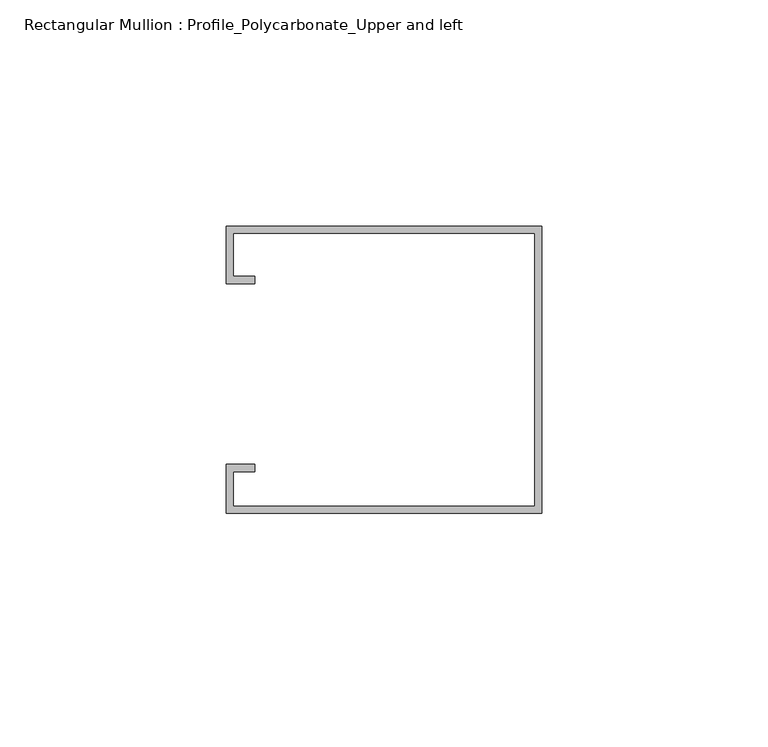
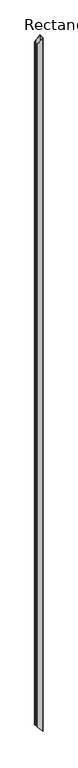
"""IFC4 building model written with IfcOpenShell, lengths in millimetres: member geometry, Rectangular Mullion : Profile_Polycarbonate_Upper and left."""

import ifcopenshell
import ifcopenshell.guid

model = None  # the IFC model being written
_history = None  # IfcOwnerHistory: only IFC2X3 demands one
_inside = {}  # id of a spatial element -> (the spatial element, [elements in it])
_under = {}  # id of a project, library or spatial element -> (it, [spatial elements below it])
_declared = {}  # id of a project -> (the project, [libraries it declares])
_typed = {}  # id of a type object -> (the type object, [elements of that type])
_made_of = {}  # id of a material, layer set ... -> (it, [elements and type objects made of it])


def new_model(schema):
    """Start an empty IFC model of exactly this schema.

    Asked for "IFC4X3", IfcOpenShell would pick the latest addendum, in which some entities
    have other attributes; the version numbers below select the first issue.
    IFC2X3 requires an IfcOwnerHistory on every rooted entity: one is made here for all.
    """
    global model, _history
    if schema == "IFC4X3":
        model = ifcopenshell.file(schema_version=(4, 3, 0, 0))
    else:
        model = ifcopenshell.file(schema=schema)
    _inside.clear()
    _under.clear()
    _declared.clear()
    _typed.clear()
    _made_of.clear()
    _history = None
    if model.schema == "IFC2X3":
        org = make("IfcOrganization", Name="unknown")
        user = make(
            "IfcPersonAndOrganization",
            ThePerson=make("IfcPerson", FamilyName="unknown"),
            TheOrganization=org,
        )
        app = make(
            "IfcApplication",
            ApplicationDeveloper=org,
            Version="unknown",
            ApplicationFullName="unknown",
            ApplicationIdentifier="unknown",
        )
        _history = make(
            "IfcOwnerHistory",
            OwningUser=user,
            OwningApplication=app,
            ChangeAction="ADDED",
            CreationDate=0,
        )
    return model


def make(cls, **values):
    """One entity of the class cls with the attributes given. An attribute that is None is left unset."""
    return model.create_entity(
        cls, **{name: value for name, value in values.items() if value is not None}
    )


def rooted(cls, **values):
    """An entity with a GlobalId (a new one), such as an element, a storey or a relation."""
    return make(cls, GlobalId=ifcopenshell.guid.new(), OwnerHistory=_history, **values)


def si_unit(unit_type, name, prefix=None):
    """IfcSIUnit, for example si_unit("LENGTHUNIT", "METRE", prefix="MILLI")."""
    return make("IfcSIUnit", UnitType=unit_type, Prefix=prefix, Name=name)


def assignment(units):
    """IfcUnitAssignment: the units of a project."""
    return None if units is None else make("IfcUnitAssignment", Units=units)


def point(xyz):
    """IfcCartesianPoint."""
    return None if xyz is None else make("IfcCartesianPoint", Coordinates=xyz)


def direction(xyz):
    """IfcDirection."""
    return None if xyz is None else make("IfcDirection", DirectionRatios=xyz)


def frame(location, z_axis=None, x_axis=None):
    """IfcAxis2Placement3D, a coordinate frame: its origin and axes. An axis left out is left unset."""
    return make(
        "IfcAxis2Placement3D",
        Location=point(location),
        Axis=direction(z_axis),
        RefDirection=direction(x_axis),
    )


def origin():
    """The frame at (0, 0, 0) with its axes left unset."""
    return frame((0.0, 0.0, 0.0))


def place(relative_to, where):
    """IfcLocalPlacement: puts the frame where relative to a parent placement (None: the world)."""
    return make(
        "IfcLocalPlacement", PlacementRelTo=relative_to, RelativePlacement=where
    )


def context(
    kind, dimensions, precision=None, world=None, true_north=None, identifier=None
):
    """IfcGeometricRepresentationContext, for example the 3D "Model" context."""
    return make(
        "IfcGeometricRepresentationContext",
        ContextIdentifier=identifier,
        ContextType=kind,
        CoordinateSpaceDimension=dimensions,
        Precision=precision,
        WorldCoordinateSystem=world,
        TrueNorth=true_north,
    )


def project(units=None, contexts=None):
    """IfcProject with its units and contexts."""
    return rooted(
        "IfcProject",
        Name="project",
        RepresentationContexts=contexts,
        UnitsInContext=assignment(units),
    )


def spatial(cls, under=None, at=None, **own):
    """A site, building, storey or space (cls), placed at a placement, below another one or the project."""
    s = rooted(cls, ObjectPlacement=at, **own)
    if under is not None:
        _under.setdefault(under.id(), (under, []))[1].append(s)
    return s


def faces_of(points, faces, orient=None, outer=None):
    """IfcFace entities. A face is a list of loops; a loop is a list of indices into points, from 0.

    orient and outer hold one flag for each loop. By default every Orientation is true, the
    first loop of a face is its IfcFaceOuterBound and the others are IfcFaceBound.
    """
    made = []
    for i, loops in enumerate(faces):
        bounds = []
        for j, loop in enumerate(loops):
            is_outer = j == 0 if outer is None else outer[i][j]
            bounds.append(
                make(
                    "IfcFaceOuterBound" if is_outer else "IfcFaceBound",
                    Bound=make("IfcPolyLoop", Polygon=[points[k] for k in loop]),
                    Orientation=True if orient is None else orient[i][j],
                )
            )
        made.append(make("IfcFace", Bounds=bounds))
    return made


def faceted_brep(points, faces, orient=None, outer=None, voids=None):
    """IfcFacetedBrep: a solid bounded by flat faces; with voids (closed shells), ...WithVoids."""
    shared = [point(p) for p in points]
    hull = make("IfcClosedShell", CfsFaces=faces_of(shared, faces, orient, outer))
    if voids is None:
        return make("IfcFacetedBrep", Outer=hull)
    return make(
        "IfcFacetedBrepWithVoids",
        Outer=hull,
        Voids=[
            make(cls, CfsFaces=faces_of(shared, fs, o, b)) for cls, fs, o, b in voids
        ],
    )


def shape(context_of_items, identifier, shape_type, items):
    """IfcShapeRepresentation: the items that make up one representation, for example the "Body"."""
    return make(
        "IfcShapeRepresentation",
        ContextOfItems=context_of_items,
        RepresentationIdentifier=identifier,
        RepresentationType=shape_type,
        Items=items,
    )


def source(mapping_origin, context_of_items, identifier, shape_type, items):
    """IfcRepresentationMap: a shape defined once, which mapped items show again and again."""
    return make(
        "IfcRepresentationMap",
        MappingOrigin=mapping_origin,
        MappedRepresentation=shape(context_of_items, identifier, shape_type, items),
    )


def transform(
    local_origin,
    x_axis=None,
    y_axis=None,
    z_axis=None,
    scale=None,
    scale2=None,
    scale3=None,
    uniform=True,
):
    """IfcCartesianTransformationOperator3D, or its non-uniform kind. x_axis, y_axis, z_axis: its Axis1, 2, 3."""
    if uniform:
        return make(
            "IfcCartesianTransformationOperator3D",
            Axis1=direction(x_axis),
            Axis2=direction(y_axis),
            LocalOrigin=point(local_origin),
            Scale=scale,
            Axis3=direction(z_axis),
        )
    return make(
        "IfcCartesianTransformationOperator3DnonUniform",
        Axis1=direction(x_axis),
        Axis2=direction(y_axis),
        LocalOrigin=point(local_origin),
        Scale=scale,
        Axis3=direction(z_axis),
        Scale2=scale2,
        Scale3=scale3,
    )


def mapped(mapping_source, mapping_target):
    """IfcMappedItem: shows the shape of a source again, moved by a transform."""
    return make(
        "IfcMappedItem", MappingSource=mapping_source, MappingTarget=mapping_target
    )


def made_of(thing, what):
    """Note that an element or type object is made of a material, layer set ...; save() writes the relation."""
    if what is not None:
        _made_of.setdefault(what.id(), (what, []))[1].append(thing)
    return thing


def element(
    cls,
    number,
    at=None,
    inside=None,
    cuts=None,
    type_object=None,
    material=None,
    context=None,
    identifier="Body",
    shape_type=None,
    held_by="IfcProductDefinitionShape",
    body=None,
    shapes=None,
    **own,
):
    """One element of the class cls, such as IfcWall. Its Tag is "e" and its number.

    at: its placement. inside: the storey or other place that contains it. cuts: it is an
    opening in that element (IfcRelVoidsElement). A single representation is given by context,
    identifier, shape_type and body (its items); several are given by shapes. held_by: the class
    of the entity that holds the representations. save() writes the other relations.
    """
    e = rooted(cls, Tag="e%d" % number, ObjectPlacement=at, **own)
    if body is not None:
        shapes = [shape(context, identifier, shape_type, body)]
    if shapes is not None:
        e.Representation = make(held_by, Representations=shapes)
    if inside is not None:
        _inside.setdefault(inside.id(), (inside, []))[1].append(e)
    if cuts is not None:
        rooted(
            "IfcRelVoidsElement", RelatingBuildingElement=cuts, RelatedOpeningElement=e
        )
    if type_object is not None:
        _typed.setdefault(type_object.id(), (type_object, []))[1].append(e)
    return made_of(e, material)


def aggregate(whole, parts):
    """IfcRelAggregates: a whole, such as a stair, and the parts it consists of."""
    return rooted("IfcRelAggregates", RelatingObject=whole, RelatedObjects=parts)


def save(model, path):
    """Write the relations noted so far, then the file.

    IfcRelAggregates (storeys below a building ...), IfcRelContainedInSpatialStructure (elements
    in a storey), IfcRelDefinesByType, IfcRelAssociatesMaterial and IfcRelDeclares: one each for
    every whole, place, type object, material and project.
    """
    for whole, parts in _under.values():
        aggregate(whole, parts)
    for where, things in _inside.values():
        rooted(
            "IfcRelContainedInSpatialStructure",
            RelatedElements=things,
            RelatingStructure=where,
        )
    for kind, things in _typed.values():
        rooted("IfcRelDefinesByType", RelatedObjects=things, RelatingType=kind)
    for what, things in _made_of.values():
        rooted("IfcRelAssociatesMaterial", RelatedObjects=things, RelatingMaterial=what)
    for by, libraries in _declared.values():
        rooted("IfcRelDeclares", RelatingContext=by, RelatedDefinitions=libraries)
    model.write(path)


def rectangular_mullion_profile_polycarbonate_upper_and_left_9a5e59f4(model_context):
    return source(origin(), model_context, "Body", "Brep", [
        faceted_brep([(-69.85, 32.7, -64.2712818), (0.0, 32.7, 0.0), (0.0, 32.7, -9272.8682286), (-69.85, 32.7, -9196.9552802), (-69.85, 20.0, -64.2712818), (-69.85, 20.0, -9196.9552802), (-63.5, 20.0, -58.428438), (-63.5, 20.0, -9203.8564573), (-63.5, 21.5875, -58.428438), (-63.5, 21.5875, -9203.8564573), (-68.2625, 21.5875, -62.8105708), (-68.2625, 21.5875, -9198.6805745), (-68.2625, 31.1125, -62.8105708), (-68.2625, 31.1125, -9198.6805745), (-1.5875, 31.1125, -1.4607109), (-1.5875, 31.1125, -9271.1429343), (-1.5875, -29.2125, -1.4607109), (-1.5875, -29.2125, -9271.1429343), (-68.2625, -29.2125, -62.8105708), (-68.2625, -29.2125, -9198.6805745), (-68.2625, -21.5875, -62.8105708), (-68.2625, -21.5875, -9198.6805745), (-63.5, -21.5875, -58.428438), (-63.5, -21.5875, -9203.8564573), (-63.5, -20.0, -58.428438), (-63.5, -20.0, -9203.8564573), (-69.85, -20.0, -64.2712818), (-69.85, -20.0, -9196.9552802), (-69.85, -30.8, -64.2712818), (-69.85, -30.8, -9196.9552802), (0.0, -30.8, 0.0), (0.0, -30.8, -9272.8682286)], [[[0, 1, 2, 3]], [[4, 0, 3, 5]], [[6, 4, 5, 7]], [[8, 6, 7, 9]], [[10, 8, 9, 11]], [[12, 10, 11, 13]], [[14, 12, 13, 15]], [[16, 14, 15, 17]], [[18, 16, 17, 19]], [[20, 18, 19, 21]], [[22, 20, 21, 23]], [[24, 22, 23, 25]], [[26, 24, 25, 27]], [[28, 26, 27, 29]], [[30, 28, 29, 31]], [[1, 30, 31, 2]], [[1, 0, 4, 6, 8, 10, 12, 14, 16, 18, 20, 22, 24, 26, 28, 30]], [[2, 31, 29, 27, 25, 23, 21, 19, 17, 15, 13, 11, 9, 7, 5, 3]]]),
    ])


if __name__ == "__main__":
    model = new_model("IFC4")
    model_context = context("Model", 3, world=origin())
    ifc_project = project(units=[si_unit("LENGTHUNIT", "METRE", prefix="MILLI")], contexts=[model_context])
    site = spatial("IfcSite", under=ifc_project)
    building = spatial("IfcBuilding", under=site)
    placement = place(None, origin())
    rectangular_mullion_profile_polycarbonate_upper_and_left_shape = rectangular_mullion_profile_polycarbonate_upper_and_left_9a5e59f4(model_context)
    element("IfcMember", 1, ObjectType="Rectangular Mullion : Profile_Polycarbonate_Upper and left", at=placement, inside=building, context=model_context, shape_type="MappedRepresentation", body=[
        mapped(rectangular_mullion_profile_polycarbonate_upper_and_left_shape, transform((0.0, 0.0, 0.0), x_axis=(1.0, 0.0, 0.0), y_axis=(0.0, 1.0, 0.0), z_axis=(0.0, 0.0, 1.0))),
    ])
    save(model, "model.ifc")

# Revit data of these elements
# Type "Rectangular Mullion : Profile_Polycarbonate_Upper and left"
#   built-in parameter 1007322 = 0.208333 (stored number, unit not read)
#   built-in parameter 1007321 = 0.00520833 (stored number, unit not read)
#   built-in parameter 1007320 = 0 (stored number, unit not read)
# Element 1 (IfcMember, "Rectangular Mullion : Profile_Polycarbonate_Upper and left")
#   Materials on its faces: "ALUMINUM PROFILE AT POLYCARBONATE PANEL"
# Materials
#   "ALUMINUM PROFILE AT POLYCARBONATE PANEL": class "Metal", colour RGB 244 244 244, transparency 0, Description = "Aluminum 6061", Cost = 0
